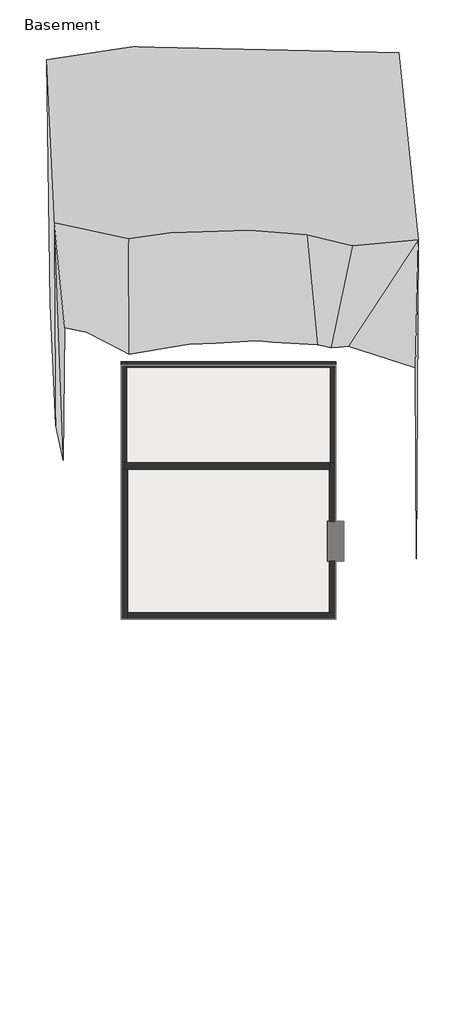
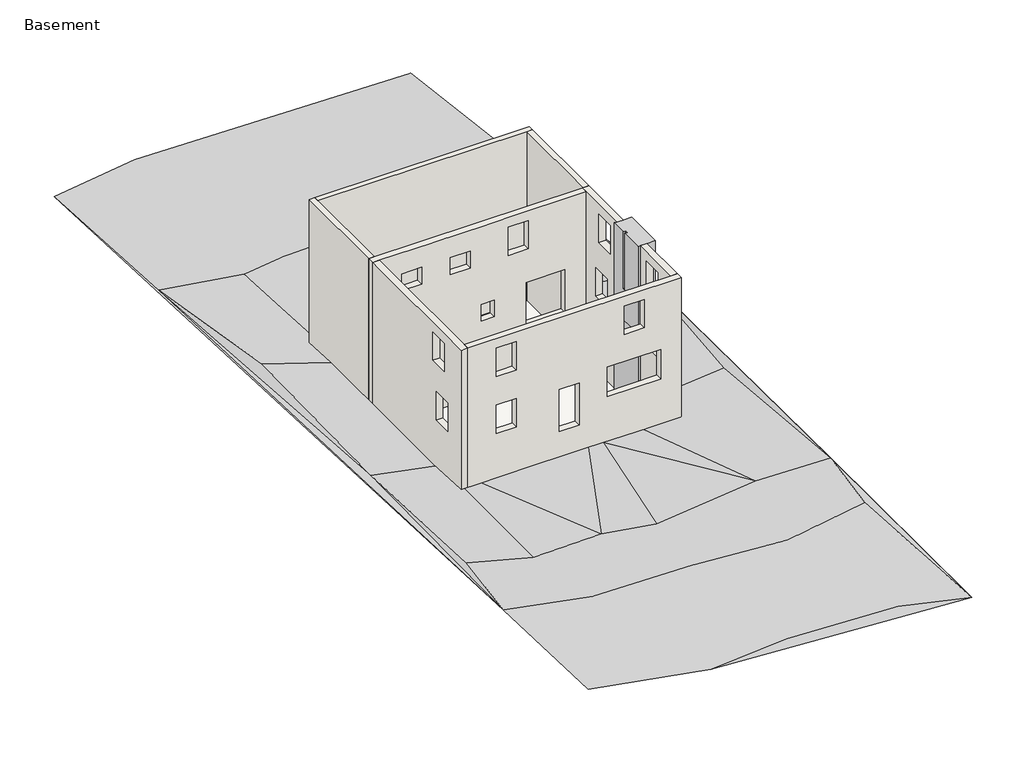
# One storey: 8 walls, 4 proxies, 2 slabs.
"""IFC4 building model written with IfcOpenShell, lengths in millimetres."""

import ifcopenshell
import ifcopenshell.guid

model = None  # the IFC model being written
_history = None  # IfcOwnerHistory: only IFC2X3 demands one
_inside = {}  # id of a spatial element -> (the spatial element, [elements in it])
_under = {}  # id of a project, library or spatial element -> (it, [spatial elements below it])
_declared = {}  # id of a project -> (the project, [libraries it declares])
_typed = {}  # id of a type object -> (the type object, [elements of that type])
_made_of = {}  # id of a material, layer set ... -> (it, [elements and type objects made of it])


def new_model(schema):
    """Start an empty IFC model of exactly this schema.

    Asked for "IFC4X3", IfcOpenShell would pick the latest addendum, in which some entities
    have other attributes; the version numbers below select the first issue.
    IFC2X3 requires an IfcOwnerHistory on every rooted entity: one is made here for all.
    """
    global model, _history
    if schema == "IFC4X3":
        model = ifcopenshell.file(schema_version=(4, 3, 0, 0))
    else:
        model = ifcopenshell.file(schema=schema)
    _inside.clear()
    _under.clear()
    _declared.clear()
    _typed.clear()
    _made_of.clear()
    _history = None
    if model.schema == "IFC2X3":
        org = make("IfcOrganization", Name="unknown")
        user = make(
            "IfcPersonAndOrganization",
            ThePerson=make("IfcPerson", FamilyName="unknown"),
            TheOrganization=org,
        )
        app = make(
            "IfcApplication",
            ApplicationDeveloper=org,
            Version="unknown",
            ApplicationFullName="unknown",
            ApplicationIdentifier="unknown",
        )
        _history = make(
            "IfcOwnerHistory",
            OwningUser=user,
            OwningApplication=app,
            ChangeAction="ADDED",
            CreationDate=0,
        )
    return model


def make(cls, **values):
    """One entity of the class cls with the attributes given. An attribute that is None is left unset."""
    return model.create_entity(
        cls, **{name: value for name, value in values.items() if value is not None}
    )


def rooted(cls, **values):
    """An entity with a GlobalId (a new one), such as an element, a storey or a relation."""
    return make(cls, GlobalId=ifcopenshell.guid.new(), OwnerHistory=_history, **values)


def si_unit(unit_type, name, prefix=None):
    """IfcSIUnit, for example si_unit("LENGTHUNIT", "METRE", prefix="MILLI")."""
    return make("IfcSIUnit", UnitType=unit_type, Prefix=prefix, Name=name)


def assignment(units):
    """IfcUnitAssignment: the units of a project."""
    return None if units is None else make("IfcUnitAssignment", Units=units)


def point(xyz):
    """IfcCartesianPoint."""
    return None if xyz is None else make("IfcCartesianPoint", Coordinates=xyz)


def direction(xyz):
    """IfcDirection."""
    return None if xyz is None else make("IfcDirection", DirectionRatios=xyz)


def frame(location, z_axis=None, x_axis=None):
    """IfcAxis2Placement3D, a coordinate frame: its origin and axes. An axis left out is left unset."""
    return make(
        "IfcAxis2Placement3D",
        Location=point(location),
        Axis=direction(z_axis),
        RefDirection=direction(x_axis),
    )


def origin():
    """The frame at (0, 0, 0) with its axes left unset."""
    return frame((0.0, 0.0, 0.0))


def place(relative_to, where):
    """IfcLocalPlacement: puts the frame where relative to a parent placement (None: the world)."""
    return make(
        "IfcLocalPlacement", PlacementRelTo=relative_to, RelativePlacement=where
    )


def context(
    kind, dimensions, precision=None, world=None, true_north=None, identifier=None
):
    """IfcGeometricRepresentationContext, for example the 3D "Model" context."""
    return make(
        "IfcGeometricRepresentationContext",
        ContextIdentifier=identifier,
        ContextType=kind,
        CoordinateSpaceDimension=dimensions,
        Precision=precision,
        WorldCoordinateSystem=world,
        TrueNorth=true_north,
    )


def project(units=None, contexts=None):
    """IfcProject with its units and contexts."""
    return rooted(
        "IfcProject",
        Name="project",
        RepresentationContexts=contexts,
        UnitsInContext=assignment(units),
    )


def spatial(cls, under=None, at=None, **own):
    """A site, building, storey or space (cls), placed at a placement, below another one or the project."""
    s = rooted(cls, ObjectPlacement=at, **own)
    if under is not None:
        _under.setdefault(under.id(), (under, []))[1].append(s)
    return s


def polyline(points):
    """IfcPolyline through the points."""
    return make("IfcPolyline", Points=[point(p) for p in points])


def point_list(points):
    """IfcCartesianPointList2D or 3D."""
    cls = (
        "IfcCartesianPointList2D" if len(points[0]) == 2 else "IfcCartesianPointList3D"
    )
    return make(cls, CoordList=points)


def outline(outer, holes=None, kind="AREA"):
    """IfcArbitraryClosedProfileDef: a profile drawn as a closed curve; with holes, ...WithVoids."""
    if holes is None:
        return make("IfcArbitraryClosedProfileDef", ProfileType=kind, OuterCurve=outer)
    return make(
        "IfcArbitraryProfileDefWithVoids",
        ProfileType=kind,
        OuterCurve=outer,
        InnerCurves=holes,
    )


def extrude(swept, where, along, depth):
    """IfcExtrudedAreaSolid: the profile swept, set in the frame where, extruded along a direction by depth."""
    return make(
        "IfcExtrudedAreaSolid",
        SweptArea=swept,
        Position=where,
        ExtrudedDirection=direction(along),
        Depth=depth,
    )


def faces_of(points, faces, orient=None, outer=None):
    """IfcFace entities. A face is a list of loops; a loop is a list of indices into points, from 0.

    orient and outer hold one flag for each loop. By default every Orientation is true, the
    first loop of a face is its IfcFaceOuterBound and the others are IfcFaceBound.
    """
    made = []
    for i, loops in enumerate(faces):
        bounds = []
        for j, loop in enumerate(loops):
            is_outer = j == 0 if outer is None else outer[i][j]
            bounds.append(
                make(
                    "IfcFaceOuterBound" if is_outer else "IfcFaceBound",
                    Bound=make("IfcPolyLoop", Polygon=[points[k] for k in loop]),
                    Orientation=True if orient is None else orient[i][j],
                )
            )
        made.append(make("IfcFace", Bounds=bounds))
    return made


def faceted_brep(points, faces, orient=None, outer=None, voids=None):
    """IfcFacetedBrep: a solid bounded by flat faces; with voids (closed shells), ...WithVoids."""
    shared = [point(p) for p in points]
    hull = make("IfcClosedShell", CfsFaces=faces_of(shared, faces, orient, outer))
    if voids is None:
        return make("IfcFacetedBrep", Outer=hull)
    return make(
        "IfcFacetedBrepWithVoids",
        Outer=hull,
        Voids=[
            make(cls, CfsFaces=faces_of(shared, fs, o, b)) for cls, fs, o, b in voids
        ],
    )


def triangles(points, corners, closed=None, point_numbers=None):
    """IfcTriangulatedFaceSet: each triangle names its three corners, points numbered from 1."""
    return make(
        "IfcTriangulatedFaceSet",
        Coordinates=point_list(points),
        Closed=closed,
        CoordIndex=corners,
        PnIndex=point_numbers,
    )


def shape(context_of_items, identifier, shape_type, items):
    """IfcShapeRepresentation: the items that make up one representation, for example the "Body"."""
    return make(
        "IfcShapeRepresentation",
        ContextOfItems=context_of_items,
        RepresentationIdentifier=identifier,
        RepresentationType=shape_type,
        Items=items,
    )


def source(mapping_origin, context_of_items, identifier, shape_type, items):
    """IfcRepresentationMap: a shape defined once, which mapped items show again and again."""
    return make(
        "IfcRepresentationMap",
        MappingOrigin=mapping_origin,
        MappedRepresentation=shape(context_of_items, identifier, shape_type, items),
    )


def transform(
    local_origin,
    x_axis=None,
    y_axis=None,
    z_axis=None,
    scale=None,
    scale2=None,
    scale3=None,
    uniform=True,
):
    """IfcCartesianTransformationOperator3D, or its non-uniform kind. x_axis, y_axis, z_axis: its Axis1, 2, 3."""
    if uniform:
        return make(
            "IfcCartesianTransformationOperator3D",
            Axis1=direction(x_axis),
            Axis2=direction(y_axis),
            LocalOrigin=point(local_origin),
            Scale=scale,
            Axis3=direction(z_axis),
        )
    return make(
        "IfcCartesianTransformationOperator3DnonUniform",
        Axis1=direction(x_axis),
        Axis2=direction(y_axis),
        LocalOrigin=point(local_origin),
        Scale=scale,
        Axis3=direction(z_axis),
        Scale2=scale2,
        Scale3=scale3,
    )


def mapped(mapping_source, mapping_target):
    """IfcMappedItem: shows the shape of a source again, moved by a transform."""
    return make(
        "IfcMappedItem", MappingSource=mapping_source, MappingTarget=mapping_target
    )


def made_of(thing, what):
    """Note that an element or type object is made of a material, layer set ...; save() writes the relation."""
    if what is not None:
        _made_of.setdefault(what.id(), (what, []))[1].append(thing)
    return thing


def element(
    cls,
    number,
    at=None,
    inside=None,
    cuts=None,
    type_object=None,
    material=None,
    context=None,
    identifier="Body",
    shape_type=None,
    held_by="IfcProductDefinitionShape",
    body=None,
    shapes=None,
    **own,
):
    """One element of the class cls, such as IfcWall. Its Tag is "e" and its number.

    at: its placement. inside: the storey or other place that contains it. cuts: it is an
    opening in that element (IfcRelVoidsElement). A single representation is given by context,
    identifier, shape_type and body (its items); several are given by shapes. held_by: the class
    of the entity that holds the representations. save() writes the other relations.
    """
    e = rooted(cls, Tag="e%d" % number, ObjectPlacement=at, **own)
    if body is not None:
        shapes = [shape(context, identifier, shape_type, body)]
    if shapes is not None:
        e.Representation = make(held_by, Representations=shapes)
    if inside is not None:
        _inside.setdefault(inside.id(), (inside, []))[1].append(e)
    if cuts is not None:
        rooted(
            "IfcRelVoidsElement", RelatingBuildingElement=cuts, RelatedOpeningElement=e
        )
    if type_object is not None:
        _typed.setdefault(type_object.id(), (type_object, []))[1].append(e)
    return made_of(e, material)


def aggregate(whole, parts):
    """IfcRelAggregates: a whole, such as a stair, and the parts it consists of."""
    return rooted("IfcRelAggregates", RelatingObject=whole, RelatedObjects=parts)


def save(model, path):
    """Write the relations noted so far, then the file.

    IfcRelAggregates (storeys below a building ...), IfcRelContainedInSpatialStructure (elements
    in a storey), IfcRelDefinesByType, IfcRelAssociatesMaterial and IfcRelDeclares: one each for
    every whole, place, type object, material and project.
    """
    for whole, parts in _under.values():
        aggregate(whole, parts)
    for where, things in _inside.values():
        rooted(
            "IfcRelContainedInSpatialStructure",
            RelatedElements=things,
            RelatingStructure=where,
        )
    for kind, things in _typed.values():
        rooted("IfcRelDefinesByType", RelatedObjects=things, RelatingType=kind)
    for what, things in _made_of.values():
        rooted("IfcRelAssociatesMaterial", RelatedObjects=things, RelatingMaterial=what)
    for by, libraries in _declared.values():
        rooted("IfcRelDeclares", RelatingContext=by, RelatedDefinitions=libraries)
    model.write(path)


def existing_fireplace_existing_fireplace_063a625f(model_context):
    return source(origin(), model_context, "Body", "Brep", [
        faceted_brep([(4450.2196932, 434.2888758, 5486.4), (4069.2196932, 434.2888758, 5486.4), (3764.4196932, 434.2888758, 5486.4), (3662.8196932, 434.2888758, 5486.4), (3662.8196932, -276.9111242, 5486.4), (3767.2567114, -276.9111242, 5486.4), (3767.2567114, -403.9111242, 5486.4), (3662.8196932, -403.9111242, 5486.4), (3662.8196932, -1445.3111242, 5486.4), (3764.4196932, -1445.3111242, 5486.4), (4069.2196932, -1445.3111242, 5486.4), (4450.2196932, -1445.3111242, 5486.4), (4450.2196932, 434.2888758, -2667.0), (4450.2196932, -1445.3111242, -2667.0), (4069.2196932, -1445.3111242, -2667.0), (3764.4196932, -1445.3111242, -2667.0), (3662.8196932, -1445.3111242, -2667.0), (3662.8196932, 434.2888758, -2667.0), (3764.4196932, 434.2888758, -2667.0), (4069.2196932, 434.2888758, -2667.0), (3662.8196932, -403.9111242, 2743.2), (3662.8196932, -276.9111242, 2743.2), (3662.8196932, 154.8888758, 0.0), (3662.8196932, 154.8888758, 1219.2), (3662.8196932, -1165.9111242, 1219.2), (3662.8196932, -1165.9111242, 0.0), (4145.4196932, -20.7631592, 1219.2), (4145.4196932, -990.2590891, 1219.2), (4145.4196932, -990.2590891, 0.0), (4145.4196932, -20.7631592, 0.0), (3767.2567114, -403.9111242, 2743.2), (3767.2567114, -276.9111242, 2743.2)], [[[0, 1, 2, 3, 4, 5, 6, 7, 8, 9, 10, 11]], [[12, 13, 14, 15, 16, 17, 18, 19]], [[3, 2, 1, 0, 12, 19, 18, 17]], [[3, 17, 16, 8, 7, 20, 21, 4], [22, 23, 24, 25]], [[11, 10, 9, 8, 16, 15, 14, 13]], [[0, 11, 13, 12]], [[24, 23, 26, 27]], [[25, 24, 27, 28]], [[27, 26, 29, 28]], [[23, 22, 29, 26]], [[22, 25, 28, 29]], [[6, 30, 20, 7]], [[31, 5, 4, 21]], [[30, 31, 21, 20]], [[30, 6, 5, 31]]]),
    ])


model = new_model("IFC4")

# Units and contexts
model_context = context("Model", 3, world=origin())
ifc_project = project(units=[si_unit("LENGTHUNIT", "METRE", prefix="MILLI")], contexts=[model_context])

# Site, building, storey
site = spatial("IfcSite", under=ifc_project)
building = spatial("IfcBuilding", under=site)
storey = spatial("IfcBuildingStorey", under=building, Name="Basement", Elevation=-2667.0)

# Proxies
placement = place(None, origin())
element("IfcBuildingElementProxy", 1, Name="Building Element Proxy", at=placement, inside=storey, context=model_context, shape_type="Tessellation", body=[
    triangles([(-9474.14729, 22003.2871765, -1727.1999516), (-8916.1412338, -12566.1132111, -939.7999758), (-8632.7724838, -18803.3999359, -1092.1999758), (-3754.3850807, -20036.8885986, -1092.1999758), (7677.2023224, -20906.8378235, -1092.1999758), (7936.7585724, 13587.9496765, -1752.6), (7012.0400162, 22339.8364014, -1727.1999516), (-5437.1349838, 22620.8239014, -1727.1999516), (4069.2196426, 434.2888621, -1346.1999516), (4450.2196426, 434.2888621, -1346.1999516), (4450.2196426, -349.5066825, -1346.1999516), (4450.2196426, -1445.3110531, -1346.1999516), (4069.2196426, -1445.3110531, -1346.1999516), (4069.2196426, -2313.9084709, -1346.1999516), (4069.2196426, -4163.1110046, -1246.6980309), (3428.5651428, -4163.1110046, -1250.4688763), (2349.5500454, -4163.1110046, -1257.7835461), (502.5996998, -4163.1110046, -1235.211668), (-175.7374563, -4163.1110046, -1228.3558365), (-2922.786422, -4163.1110046, -1226.4072636), (-5055.1879486, -4163.1110046, -1242.8984081), (-5852.784613, -4163.1110046, -1243.6517052), (-5989.1803574, -4163.1110046, -1240.8027512), (-5989.1803574, -2711.9263275, -1314.8636375), (-5989.1803574, -2124.4043404, -1346.1999516), (-5989.1803574, 3152.0889954, -1346.1999516), (-5989.1803574, 4989.0600082, -1346.1999516), (-5989.1803574, 6156.3282944, -1346.1999516), (-5989.1803574, 7724.0889954, -1429.2445919), (-5611.7969971, 7724.0889954, -1439.6358181), (-2815.8938187, 7724.0889954, -1415.0254017), (-2474.4123367, 7724.0889954, -1412.4145145), (-1876.9665367, 7724.0889954, -1411.4359406), (391.3462071, 7724.0889954, -1403.6252254), (781.867392, 7724.0889954, -1405.4288944), (3306.7437996, 7724.0889954, -1413.4377079), (3676.8014442, 7724.0889954, -1418.4369667), (4069.2196426, 7724.0889954, -1416.2554138), (4069.2196426, 7529.9159637, -1404.4058464), (4069.2196426, 6299.0253983, -1346.1999516), (4069.2196426, 3152.0889954, -1346.1999516), (-9109.81604, 14372.1750641, -1752.6), (-8549.4287338, -9013.2876297, -939.7999758), (-8523.2349838, -1401.2252266, -1346.1999516), (-8408.9349838, 7414.1625641, -1346.1999516), (-6082.4537338, -10022.9382111, -939.7999758), (-5633.19104, 13643.5125641, -1752.6), (-5382.3662338, -13518.6132111, -939.7999758), (-3671.0413307, 13924.5000641, -1752.6), (-2942.3788307, -9965.7882111, -939.7999758), (-1568.3975807, 21947.7254517, -1727.1999516), (-840.5287823, -13629.7378235, -939.7999758), (-699.241258, -10470.6132111, -939.7999758), (-109.4850414, -19700.3370483, -1092.1999758), (29.4212079, 14035.6246765, -1752.6), (2721.8210724, 13811.7871765, -1752.6), (2805.1648224, 21892.1614014, -1727.1999516), (3252.0462662, -14021.8499359, -939.7999758), (4179.1460724, -9854.6624359, -939.7999758), (4845.1025162, -19962.2745483, -1092.1999758), (4852.2462662, 13306.9621765, -1752.6), (7177.93396, -13294.7757111, -939.7999758), (7289.85271, -1961.6126781, -1346.1999516), (7543.0587662, -9965.7882111, -939.7999758), (7740.7025162, 5059.8998703, -1346.1999516)], [[46, 2, 48], [43, 46, 23], [46, 43, 2], [2, 3, 48], [2, 43, 44], [43, 23, 44], [23, 46, 22], [44, 23, 24], [46, 21, 22], [44, 24, 25], [48, 4, 52], [4, 48, 3], [48, 52, 50], [19, 53, 18], [4, 54, 52], [50, 52, 53], [21, 50, 20], [21, 46, 50], [19, 20, 50], [50, 53, 19], [53, 52, 58], [50, 46, 48], [45, 27, 28], [26, 27, 45], [44, 26, 45], [25, 26, 44], [8, 1, 42], [1, 2, 42], [42, 45, 47], [29, 45, 28], [42, 44, 45], [29, 47, 45], [42, 2, 44], [47, 30, 31], [31, 32, 49], [33, 49, 32], [47, 8, 42], [8, 47, 49], [49, 51, 8], [55, 51, 49], [47, 31, 49], [8, 51, 57], [55, 49, 33], [30, 47, 29], [58, 59, 53], [58, 54, 60], [59, 15, 16], [59, 18, 53], [16, 17, 59], [59, 17, 18], [12, 13, 14], [14, 15, 63], [58, 62, 59], [62, 60, 5], [64, 5, 65], [5, 64, 62], [60, 54, 5], [59, 62, 64], [59, 64, 15], [12, 63, 11], [12, 14, 63], [64, 63, 15], [11, 63, 10], [64, 65, 63], [62, 58, 60], [54, 4, 5], [55, 34, 35], [56, 35, 36], [55, 56, 57], [55, 35, 56], [37, 61, 36], [56, 61, 57], [56, 36, 61], [55, 57, 51], [55, 33, 34], [40, 41, 65], [10, 65, 41], [65, 10, 63], [41, 9, 10], [40, 65, 39], [39, 65, 38], [61, 6, 7], [6, 61, 38], [61, 7, 57], [65, 6, 38], [38, 61, 37], [65, 5, 6], [57, 7, 8], [52, 54, 58]], closed=False),
])
element("IfcBuildingElementProxy", 2, Name="Building Element Proxy", at=placement, inside=storey, context=model_context, shape_type="Tessellation", body=[
    triangles([(4069.2196426, 3152.0889954, -3073.5594864), (4069.2196426, 3152.0889954, -1346.1999516), (4069.2196426, 434.2888621, -3073.5594864), (4069.2196426, 434.2888621, -1346.1999516), (4450.2196426, 434.2888621, -3073.5594864), (4450.2196426, 434.2888621, -1346.1999516), (4450.2196426, -349.5066825, -3073.5594864), (4450.2196426, -349.5066825, -1346.1999516), (4450.2196426, -1445.3110531, -3073.5594864), (4450.2196426, -1445.3110531, -1346.1999516), (4069.2196426, -1445.3110531, -3073.5594864), (4069.2196426, -1445.3110531, -1346.1999516), (4069.2196426, -2313.9084709, -3073.5594864), (4069.2196426, -2313.9084709, -1346.1999516), (4069.2196426, -4163.1110046, -3073.5594864), (4069.2196426, -4163.1110046, -1246.6980309), (3428.5651428, -4163.1110046, -3073.5594864), (3428.5651428, -4163.1110046, -1250.4688763), (2349.5500454, -4163.1110046, -3073.5594864), (2349.5500454, -4163.1110046, -1257.7835461), (502.5996998, -4163.1110046, -3073.5594864), (502.5996998, -4163.1110046, -1235.211668), (-175.7374563, -4163.1110046, -3073.5594864), (-175.7374563, -4163.1110046, -1228.3558365), (-2922.786422, -4163.1110046, -3073.5594864), (-2922.786422, -4163.1110046, -1226.4072636), (-5055.1879486, -4163.1110046, -3073.5594864), (-5055.1879486, -4163.1110046, -1242.8984081), (-5852.784613, -4163.1110046, -3073.5594864), (-5852.784613, -4163.1110046, -1243.6517052), (-5989.1803574, -4163.1110046, -3073.5594864), (-5989.1803574, -4163.1110046, -1240.8027512), (-5989.1803574, -2711.9263275, -3073.5594864), (-5989.1803574, -2711.9263275, -1314.8636375), (-5989.1803574, -2124.4043404, -3073.5594864), (-5989.1803574, -2124.4043404, -1346.1999516), (-5989.1803574, 3152.0889954, -3073.5594864), (-5989.1803574, 3152.0889954, -1346.1999516)], [[1, 4, 2], [1, 3, 4], [3, 6, 4], [3, 5, 6], [5, 8, 6], [5, 7, 8], [7, 10, 8], [7, 9, 10], [9, 12, 10], [9, 11, 12], [11, 14, 12], [11, 13, 14], [13, 16, 14], [13, 15, 16], [15, 18, 16], [15, 17, 18], [17, 20, 18], [17, 19, 20], [19, 22, 20], [19, 21, 22], [21, 24, 22], [21, 23, 24], [23, 26, 24], [23, 25, 26], [25, 28, 26], [25, 27, 28], [27, 30, 28], [27, 29, 30], [29, 32, 30], [29, 31, 32], [31, 34, 32], [31, 33, 34], [33, 36, 34], [33, 35, 36], [35, 38, 36], [35, 37, 38]], closed=False),
    triangles([(4069.2196426, 434.2888621, -3073.5594864), (4069.2196426, 3152.0889954, -3073.5594864), (-5989.1803574, 3152.0889954, -3073.5594864), (-5989.1803574, -4163.1110046, -3073.5594864), (4069.2196426, -4163.1110046, -3073.5594864), (4069.2196426, -1445.3110531, -3073.5594864), (4450.2196426, -1445.3110531, -3073.5594864), (4450.2196426, 434.2888621, -3073.5594864)], [[4, 6, 3], [6, 4, 5], [3, 1, 2], [1, 3, 6], [6, 7, 1], [8, 1, 7]], closed=False),
])
element("IfcBuildingElementProxy", 3, Name="Building Element Proxy", at=placement, inside=storey, context=model_context, shape_type="Tessellation", body=[
    triangles([(-5989.1803574, 3152.0889954, -3073.5594864), (-5989.1803574, 3152.0889954, -1346.1999516), (-5989.1803574, 4989.0600082, -3073.5594864), (-5989.1803574, 4989.0600082, -1346.1999516), (-5989.1803574, 6156.3282944, -3073.5594864), (-5989.1803574, 6156.3282944, -1346.1999516), (-5989.1803574, 7724.0889954, -3073.5594864), (-5989.1803574, 7724.0889954, -1429.2445919), (-5611.7969971, 7724.0889954, -3073.5594864), (-5611.7969971, 7724.0889954, -1439.6358181), (-2815.8938187, 7724.0889954, -3073.5594864), (-2815.8938187, 7724.0889954, -1415.0254017), (-2474.4123367, 7724.0889954, -3073.5594864), (-2474.4123367, 7724.0889954, -1412.4145145), (-1876.9665367, 7724.0889954, -3073.5594864), (-1876.9665367, 7724.0889954, -1411.4359406), (391.3462071, 7724.0889954, -3073.5594864), (391.3462071, 7724.0889954, -1403.6252254), (781.867392, 7724.0889954, -3073.5594864), (781.867392, 7724.0889954, -1405.4288944), (3306.7437996, 7724.0889954, -3073.5594864), (3306.7437996, 7724.0889954, -1413.4377079), (3676.8014442, 7724.0889954, -3073.5594864), (3676.8014442, 7724.0889954, -1418.4369667), (4069.2196426, 7724.0889954, -3073.5594864), (4069.2196426, 7724.0889954, -1416.2554138), (4069.2196426, 7529.9159637, -3073.5594864), (4069.2196426, 7529.9159637, -1404.4058464), (4069.2196426, 6299.0253983, -3073.5594864), (4069.2196426, 6299.0253983, -1346.1999516), (4069.2196426, 3152.0889954, -3073.5594864), (4069.2196426, 3152.0889954, -1346.1999516)], [[1, 4, 2], [1, 3, 4], [3, 6, 4], [3, 5, 6], [5, 8, 6], [5, 7, 8], [7, 10, 8], [7, 9, 10], [9, 12, 10], [9, 11, 12], [11, 14, 12], [11, 13, 14], [13, 16, 14], [13, 15, 16], [15, 18, 16], [15, 17, 18], [17, 20, 18], [17, 19, 20], [19, 22, 20], [19, 21, 22], [21, 24, 22], [21, 23, 24], [23, 26, 24], [23, 25, 26], [25, 28, 26], [25, 27, 28], [27, 30, 28], [27, 29, 30], [29, 32, 30], [29, 31, 32]], closed=False),
    triangles([(-5989.1803574, 7724.0889954, -3073.5594864), (-5989.1803574, 3152.0889954, -3073.5594864), (4069.2196426, 3152.0889954, -3073.5594864), (4069.2196426, 7724.0889954, -3073.5594864)], [[1, 2, 4], [3, 4, 2]], closed=False),
])
existing_fireplace_existing_fireplace_shape = existing_fireplace_existing_fireplace_063a625f(model_context)
element("IfcBuildingElementProxy", 4, Name="Existing Fireplace : Existing Fireplace", ObjectType="Existing Fireplace : Existing Fireplace", at=placement, inside=storey, context=model_context, shape_type="MappedRepresentation", body=[
    mapped(existing_fireplace_existing_fireplace_shape, transform((0.0, 0.0, 0.0), x_axis=(1.0, 0.0, 0.0), y_axis=(0.0, 1.0, 0.0), z_axis=(0.0, 0.0, 1.0))),
])

# Slabs
element("IfcSlab", 5, ObjectType="Pad 1", at=placement, inside=storey, context=model_context, shape_type="SweptSolid", body=[
    extrude(outline(polyline([(4069.2196932, 434.2888758), (4450.2196932, 434.2888758), (4450.2196932, -1445.3111242), (4069.2196932, -1445.3111242), (4069.2196932, -4163.1111242), (-5989.1803068, -4163.1111242), (-5989.1803068, 3152.0888758), (4069.2196932, 3152.0888758), (4069.2196932, 434.2888758)])), frame((0.0, 0.0, -3073.4), z_axis=(0.0, 0.0, 1.0), x_axis=(1.0, 0.0, 0.0)), (0.0, 0.0, 1.0), 304.8),
])
element("IfcSlab", 6, ObjectType="Pad 1", at=placement, inside=storey, context=model_context, shape_type="SweptSolid", body=[
    extrude(outline(polyline([(-5989.1803068, 7724.0888758), (4069.2196932, 7724.0888758), (4069.2196932, 3152.0888758), (-5989.1803068, 3152.0888758), (-5989.1803068, 7724.0888758)])), frame((0.0, 0.0, -3073.4), z_axis=(0.0, 0.0, 1.0), x_axis=(1.0, 0.0, 0.0)), (0.0, 0.0, 1.0), 304.8),
])

# Walls
element("IfcWall", 7, ObjectType="Generic - 10\"", at=placement, inside=storey, context=model_context, shape_type="Brep", body=[
    faceted_brep([(-5735.1803068, 3152.0888758, -2667.0), (-5735.1803068, 7622.4888758, -2667.0), (-5735.1803068, 7876.4888758, -2667.0), (-5735.1803068, 7876.4888758, 5486.4), (-5735.1803068, 7622.4888758, 5486.4), (-5735.1803068, 3152.0888758, 5486.4), (-5989.1803068, 3152.0888758, -2667.0), (-5989.1803068, 3152.0888758, 5486.4), (-5989.1803068, 7876.4888758, 5486.4), (-5989.1803068, 7876.4888758, -2667.0)], [[[0, 1, 2, 3, 4, 5]], [[6, 7, 8, 9]], [[2, 1, 0, 6, 9]], [[5, 4, 3, 8, 7]], [[3, 2, 9, 8]], [[0, 5, 7, 6]]]),
])
element("IfcWall", 8, ObjectType="Generic - 10\"", at=placement, inside=storey, context=model_context, shape_type="Brep", body=[
    faceted_brep([(-5735.1803068, 7622.4888758, -2667.0), (3815.2196932, 7622.4888758, -2667.0), (4069.2196932, 7622.4888758, -2667.0), (4069.2196932, 7622.4888758, 5486.4), (3815.2196932, 7622.4888758, 5486.4), (-5735.1803068, 7622.4888758, 5486.4), (-5735.1803068, 7876.4888758, -2667.0), (-5735.1803068, 7876.4888758, 5486.4), (4069.2196932, 7876.4888758, 5486.4), (4069.2196932, 7876.4888758, -2667.0)], [[[0, 1, 2, 3, 4, 5]], [[6, 7, 8, 9]], [[2, 1, 0, 6, 9]], [[5, 4, 3, 8, 7]], [[3, 2, 9, 8]], [[0, 5, 7, 6]]]),
])
element("IfcWall", 9, ObjectType="Generic - 10\"", at=placement, inside=storey, context=model_context, shape_type="SweptSolid", body=[
    extrude(outline(polyline([(3815.2196932, 3152.0888758), (3815.2196932, 7622.4888758), (4069.2196932, 7622.4888758), (4069.2196932, 3152.0888758), (3815.2196932, 3152.0888758)])), frame((0.0, 0.0, -2667.0), z_axis=(0.0, 0.0, 1.0), x_axis=(1.0, 0.0, 0.0)), (0.0, 0.0, 1.0), 8153.4),
])
element("IfcWall", 10, ObjectType="Generic - 12\"", at=placement, inside=storey, context=model_context, shape_type="Brep", body=[
    faceted_brep([(-5989.1803068, 2847.2888758, -2667.0), (-5684.3803068, 2847.2888758, -2667.0), (3764.4196932, 2847.2888758, -2667.0), (3764.4196932, 2847.2888758, 5486.4), (56.0196932, 2847.2888758, 5486.4), (-70.9803068, 2847.2888758, 5486.4), (-680.5803068, 2847.2888758, 5486.4), (-807.5803068, 2847.2888758, 5486.4), (-3169.7803068, 2847.2888758, 5486.4), (-3296.7803068, 2847.2888758, 5486.4), (-5684.3803068, 2847.2888758, 5486.4), (-5989.1803068, 2847.2888758, 5486.4), (1021.2196932, 2847.2888758, 0.0), (1021.2196932, 2847.2888758, 2057.4), (2799.2196932, 2847.2888758, 2057.4), (2799.2196932, 2847.2888758, 0.0), (-4160.3803068, 2847.2888758, 0.0), (-5023.9803068, 2847.2888758, 0.0), (-5023.9803068, 2847.2888758, 2032.0), (-4160.3803068, 2847.2888758, 2032.0), (-1036.1803068, 2847.2888758, 914.4), (-1036.1803068, 2847.2888758, 1727.2), (-426.5803068, 2847.2888758, 1727.2), (-426.5803068, 2847.2888758, 914.4), (-3919.0803068, 2847.2888758, 914.4), (-3919.0803068, 2847.2888758, 1727.2), (-3004.6803068, 2847.2888758, 1727.2), (-3004.6803068, 2847.2888758, 914.4), (208.4196932, 2847.2888758, 3657.6), (208.4196932, 2847.2888758, 5029.2), (1122.8196932, 2847.2888758, 5029.2), (1122.8196932, 2847.2888758, 3657.6), (-2433.1803068, 2847.2888758, 3657.6), (-2433.1803068, 2847.2888758, 4470.4), (-1518.7803068, 2847.2888758, 4470.4), (-1518.7803068, 2847.2888758, 3657.6), (-4668.3803068, 2847.2888758, 3657.6), (-4668.3803068, 2847.2888758, 4470.4), (-3753.9803068, 2847.2888758, 4470.4), (-3753.9803068, 2847.2888758, 3657.6), (3764.4196932, 3152.0888758, -2667.0), (-5989.1803068, 3152.0888758, -2667.0), (-5989.1803068, 3152.0888758, 5486.4), (3764.4196932, 3152.0888758, 5486.4), (1021.2196932, 3152.0888758, 2057.4), (1021.2196932, 3152.0888758, 0.0), (2799.2196932, 3152.0888758, 0.0), (2799.2196932, 3152.0888758, 2057.4), (-5023.9803068, 3152.0888758, 0.0), (-4160.3803068, 3152.0888758, 0.0), (-4160.3803068, 3152.0888758, 2032.0), (-5023.9803068, 3152.0888758, 2032.0), (-1036.1803068, 3152.0888758, 1727.2), (-1036.1803068, 3152.0888758, 914.4), (-426.5803068, 3152.0888758, 914.4), (-426.5803068, 3152.0888758, 1727.2), (-3919.0803068, 3152.0888758, 1727.2), (-3919.0803068, 3152.0888758, 914.4), (-3004.6803068, 3152.0888758, 914.4), (-3004.6803068, 3152.0888758, 1727.2), (208.4196932, 3152.0888758, 5029.2), (208.4196932, 3152.0888758, 3657.6), (1122.8196932, 3152.0888758, 3657.6), (1122.8196932, 3152.0888758, 5029.2), (-2433.1803068, 3152.0888758, 4470.4), (-2433.1803068, 3152.0888758, 3657.6), (-1518.7803068, 3152.0888758, 3657.6), (-1518.7803068, 3152.0888758, 4470.4), (-4668.3803068, 3152.0888758, 4470.4), (-4668.3803068, 3152.0888758, 3657.6), (-3753.9803068, 3152.0888758, 3657.6), (-3753.9803068, 3152.0888758, 4470.4)], [[[0, 1, 2, 3, 4, 5, 6, 7, 8, 9, 10, 11], [12, 13, 14, 15], [16, 17, 18, 19], [20, 21, 22, 23], [24, 25, 26, 27], [28, 29, 30, 31], [32, 33, 34, 35], [36, 37, 38, 39]], [[40, 41, 42, 43], [44, 45, 46, 47], [48, 49, 50, 51], [52, 53, 54, 55], [56, 57, 58, 59], [60, 61, 62, 63], [64, 65, 66, 67], [68, 69, 70, 71]], [[2, 1, 0, 41, 40]], [[11, 10, 9, 8, 7, 6, 5, 4, 3, 43, 42]], [[0, 11, 42, 41]], [[3, 2, 40, 43]], [[44, 13, 12, 45]], [[13, 44, 47, 14]], [[14, 47, 46, 15]], [[45, 12, 15, 46]], [[17, 16, 49, 48]], [[18, 17, 48, 51]], [[19, 18, 51, 50]], [[16, 19, 50, 49]], [[53, 52, 21, 20]], [[54, 53, 20, 23]], [[55, 54, 23, 22]], [[52, 55, 22, 21]], [[57, 56, 25, 24]], [[58, 57, 24, 27]], [[59, 58, 27, 26]], [[56, 59, 26, 25]], [[60, 29, 28, 61]], [[61, 28, 31, 62]], [[62, 31, 30, 63]], [[29, 60, 63, 30]], [[33, 32, 65, 64]], [[32, 35, 66, 65]], [[35, 34, 67, 66]], [[34, 33, 64, 67]], [[37, 36, 69, 68]], [[36, 39, 70, 69]], [[39, 38, 71, 70]], [[38, 37, 68, 71]]]),
])
element("IfcWall", 11, ObjectType="Generic - 12\"", at=placement, inside=storey, context=model_context, shape_type="Brep", body=[
    faceted_brep([(-5684.3803068, -4163.1111242, -2667.0), (-5684.3803068, -3858.3111242, -2667.0), (-5684.3803068, 2847.2888758, -2667.0), (-5684.3803068, 2847.2888758, 5486.4), (-5684.3803068, 1450.2888758, 5486.4), (-5684.3803068, 1323.2888758, 5486.4), (-5684.3803068, -3858.3111242, 5486.4), (-5684.3803068, -4163.1111242, 5486.4), (-5684.3803068, -3096.3111242, 914.4), (-5684.3803068, -3096.3111242, 2286.0), (-5684.3803068, -2181.9111242, 2286.0), (-5684.3803068, -2181.9111242, 914.4), (-5684.3803068, -2842.3111242, 3657.6), (-5684.3803068, -2842.3111242, 5029.2), (-5684.3803068, -1927.9111242, 5029.2), (-5684.3803068, -1927.9111242, 3657.6), (-5989.1803068, 2847.2888758, -2667.0), (-5989.1803068, -4163.1111242, -2667.0), (-5989.1803068, -4163.1111242, 5486.4), (-5989.1803068, 2847.2888758, 5486.4), (-5989.1803068, -3096.3111242, 2286.0), (-5989.1803068, -3096.3111242, 914.4), (-5989.1803068, -2181.9111242, 914.4), (-5989.1803068, -2181.9111242, 2286.0), (-5989.1803068, -2842.3111242, 5029.2), (-5989.1803068, -2842.3111242, 3657.6), (-5989.1803068, -1927.9111242, 3657.6), (-5989.1803068, -1927.9111242, 5029.2)], [[[0, 1, 2, 3, 4, 5, 6, 7], [8, 9, 10, 11], [12, 13, 14, 15]], [[16, 17, 18, 19], [20, 21, 22, 23], [24, 25, 26, 27]], [[2, 1, 0, 17, 16]], [[7, 6, 5, 4, 3, 19, 18]], [[0, 7, 18, 17]], [[3, 2, 16, 19]], [[21, 20, 9, 8]], [[22, 21, 8, 11]], [[23, 22, 11, 10]], [[20, 23, 10, 9]], [[24, 13, 12, 25]], [[25, 12, 15, 26]], [[26, 15, 14, 27]], [[13, 24, 27, 14]]]),
])
element("IfcWall", 12, ObjectType="Generic - 12\"", at=placement, inside=storey, context=model_context, shape_type="Brep", body=[
    faceted_brep([(4069.2196932, -3858.3111242, -2667.0), (3764.4196932, -3858.3111242, -2667.0), (-5684.3803068, -3858.3111242, -2667.0), (-5684.3803068, -3858.3111242, 5486.4), (-2179.1803068, -3858.3111242, 5486.4), (-2052.1803068, -3858.3111242, 5486.4), (-807.5803068, -3858.3111242, 5486.4), (-680.5803068, -3858.3111242, 5486.4), (-70.9803068, -3858.3111242, 5486.4), (56.0196932, -3858.3111242, 5486.4), (3764.4196932, -3858.3111242, 5486.4), (4069.2196932, -3858.3111242, 5486.4), (-1518.7803068, -3858.3111242, 0.0), (-604.3803068, -3858.3111242, 0.0), (-604.3803068, -3858.3111242, 2032.0), (-1518.7803068, -3858.3111242, 2032.0), (-3474.5803068, -3858.3111242, 914.4), (-3474.5803068, -3858.3111242, 2286.0), (-4388.9803068, -3858.3111242, 2286.0), (-4388.9803068, -3858.3111242, 914.4), (691.0196932, -3858.3111242, 2336.8), (691.0196932, -3858.3111242, 914.4), (3129.4196932, -3858.3111242, 914.4), (3129.4196932, -3858.3111242, 2336.8), (2367.4196932, -3858.3111242, 3657.6), (2367.4196932, -3858.3111242, 5029.2), (1453.0196932, -3858.3111242, 5029.2), (1453.0196932, -3858.3111242, 3657.6), (-3474.5803068, -3858.3111242, 3657.6), (-3474.5803068, -3858.3111242, 5029.2), (-4388.9803068, -3858.3111242, 5029.2), (-4388.9803068, -3858.3111242, 3657.6), (-5684.3803068, -4163.1111242, -2667.0), (4069.2196932, -4163.1111242, -2667.0), (4069.2196932, -4163.1111242, 5486.4), (-5684.3803068, -4163.1111242, 5486.4), (-604.3803068, -4163.1111242, 0.0), (-1518.7803068, -4163.1111242, 0.0), (-1518.7803068, -4163.1111242, 2032.0), (-604.3803068, -4163.1111242, 2032.0), (-3474.5803068, -4163.1111242, 2286.0), (-3474.5803068, -4163.1111242, 914.4), (-4388.9803068, -4163.1111242, 914.4), (-4388.9803068, -4163.1111242, 2286.0), (691.0196932, -4163.1111242, 914.4), (691.0196932, -4163.1111242, 2336.8), (3129.4196932, -4163.1111242, 2336.8), (3129.4196932, -4163.1111242, 914.4), (2367.4196932, -4163.1111242, 5029.2), (2367.4196932, -4163.1111242, 3657.6), (1453.0196932, -4163.1111242, 3657.6), (1453.0196932, -4163.1111242, 5029.2), (-3474.5803068, -4163.1111242, 5029.2), (-3474.5803068, -4163.1111242, 3657.6), (-4388.9803068, -4163.1111242, 3657.6), (-4388.9803068, -4163.1111242, 5029.2)], [[[0, 1, 2, 3, 4, 5, 6, 7, 8, 9, 10, 11], [12, 13, 14, 15], [16, 17, 18, 19], [20, 21, 22, 23], [24, 25, 26, 27], [28, 29, 30, 31]], [[32, 33, 34, 35], [36, 37, 38, 39], [40, 41, 42, 43], [44, 45, 46, 47], [48, 49, 50, 51], [52, 53, 54, 55]], [[2, 1, 0, 33, 32]], [[11, 10, 9, 8, 7, 6, 5, 4, 3, 35, 34]], [[0, 11, 34, 33]], [[3, 2, 32, 35]], [[37, 36, 13, 12]], [[38, 37, 12, 15]], [[39, 38, 15, 14]], [[36, 39, 14, 13]], [[41, 40, 17, 16]], [[42, 41, 16, 19]], [[43, 42, 19, 18]], [[40, 43, 18, 17]], [[21, 44, 47, 22]], [[45, 20, 23, 46]], [[20, 45, 44, 21]], [[22, 47, 46, 23]], [[25, 24, 49, 48]], [[24, 27, 50, 49]], [[27, 26, 51, 50]], [[26, 25, 48, 51]], [[52, 29, 28, 53]], [[53, 28, 31, 54]], [[54, 31, 30, 55]], [[29, 52, 55, 30]]]),
])
element("IfcWall", 13, ObjectType="Generic - 12\"", at=placement, inside=storey, context=model_context, shape_type="Brep", body=[
    faceted_brep([(3764.4196932, 3152.0888758, -2667.0), (3764.4196932, 2847.2888758, -2667.0), (3764.4196932, 434.2888758, -2667.0), (3764.4196932, 434.2888758, 5486.4), (3764.4196932, 2847.2888758, 5486.4), (3764.4196932, 3152.0888758, 5486.4), (3764.4196932, 2085.2888758, 914.4), (3764.4196932, 2085.2888758, 2286.0), (3764.4196932, 1170.8888758, 2286.0), (3764.4196932, 1170.8888758, 914.4), (3764.4196932, 1831.2888758, 3657.6), (3764.4196932, 1831.2888758, 5029.2), (3764.4196932, 916.8888758, 5029.2), (3764.4196932, 916.8888758, 3657.6), (4069.2196932, 434.2888758, -2667.0), (4069.2196932, 3152.0888758, -2667.0), (4069.2196932, 3152.0888758, 5486.4), (4069.2196932, 434.2888758, 5486.4), (4069.2196932, 2085.2888758, 2286.0), (4069.2196932, 2085.2888758, 914.4), (4069.2196932, 1170.8888758, 914.4), (4069.2196932, 1170.8888758, 2286.0), (4069.2196932, 1831.2888758, 5029.2), (4069.2196932, 1831.2888758, 3657.6), (4069.2196932, 916.8888758, 3657.6), (4069.2196932, 916.8888758, 5029.2)], [[[0, 1, 2, 3, 4, 5], [6, 7, 8, 9], [10, 11, 12, 13]], [[14, 15, 16, 17], [18, 19, 20, 21], [22, 23, 24, 25]], [[2, 1, 0, 15, 14]], [[3, 2, 14, 17]], [[5, 4, 3, 17, 16]], [[0, 5, 16, 15]], [[19, 18, 7, 6]], [[20, 19, 6, 9]], [[21, 20, 9, 8]], [[18, 21, 8, 7]], [[22, 11, 10, 23]], [[23, 10, 13, 24]], [[24, 13, 12, 25]], [[11, 22, 25, 12]]]),
])
element("IfcWall", 14, ObjectType="Generic - 12\"", at=placement, inside=storey, context=model_context, shape_type="SweptSolid", body=[
    extrude(outline(polyline([(-1445.3111242, -2667.0), (-3858.3111242, -2667.0), (-3858.3111242, 5486.4), (-1445.3111242, 5486.4), (-1445.3111242, -2667.0)]), holes=[polyline([(-2181.9111242, 2286.0), (-3096.3111242, 2286.0), (-3096.3111242, 914.4), (-2181.9111242, 914.4), (-2181.9111242, 2286.0)]), polyline([(-1927.9111242, 3657.6), (-1927.9111242, 5029.2), (-2842.3111242, 5029.2), (-2842.3111242, 3657.6), (-1927.9111242, 3657.6)])]), frame((3764.4196932, 0.0, 0.0), z_axis=(1.0, 0.0, 0.0), x_axis=(0.0, 1.0, 0.0)), (0.0, 0.0, 1.0), 304.8),
])

save(model, "model.ifc")

# Revit data of these elements
# Project information
#   Organization Name = "G3B Press"
#   Organization Description = "Paul F. Aubin Cosulting Services, Inc."
#   Building Name = "Revit Essentials for Architecture"
#   Author = "Paul F. Aubin"
#   Author Website = "https://www.paulaubin.com"
#   Copyright = "Copyright © 2020 Paul F Aubin, all rights reserved"
#   Project Issue Date = "8/1/2020"
#   Project Status = "Design Development"
#   Client Name = "Column Grids and Structural Layout"
#   Project Address = "789 Main ST\nAnytown, IL 60000"
#   Project Name = "06 Residential"
#   Project Number = "2020.03A"
# Type "Pad 1"
#   Layers, outside or top first: 1' - 0" no material (function 1)
# Type "Generic - 10\""
#   Assembly Code = "B2010"
#   Layers, outside or top first: 0' - 10" no material (function 1)
# Type "Generic - 12\""
#   Assembly Code = "B2010"
#   Layers, outside or top first: 1' - 0" no material (function 1)
# Elements 1, 2, 3 (IfcBuildingElementProxy)
#   Material = none
#   Phase Created = New Construction
# Element 4 (IfcBuildingElementProxy, "Existing Fireplace : Existing Fireplace")
#   Phase Created = Existing
# Elements 5, 6 (IfcSlab, "Pad 1")
#   built-in parameter 1012502 = -0.333333 (stored number, unit not read)
#   Phase Created = New Construction
# Elements 7, 8, 9 (IfcWall, "Generic - 10\"")
#   Top Offset = 0' - 0"
#   Base Offset = 0' - 0"
#   wall height = 26' - 9"
#   Phase Created = New Construction
#   Base Constraint = Basement
#   Top Constraint = Roof
#   Materials on its faces: "Default Wall"
# Elements 10, 11, 12, 13, 14 (IfcWall, "Generic - 12\"")
#   Top Offset = 0' - 0"
#   Base Offset = 0' - 0"
#   wall height = 26' - 9"
#   Phase Created = Existing
#   Base Constraint = Basement
#   Top Constraint = Roof
#   Materials on its faces: "Default Wall"
# Materials
#   "Default Wall": class "Miscellaneous", colour RGB 128 128 128, transparency 0, Cost = 0
